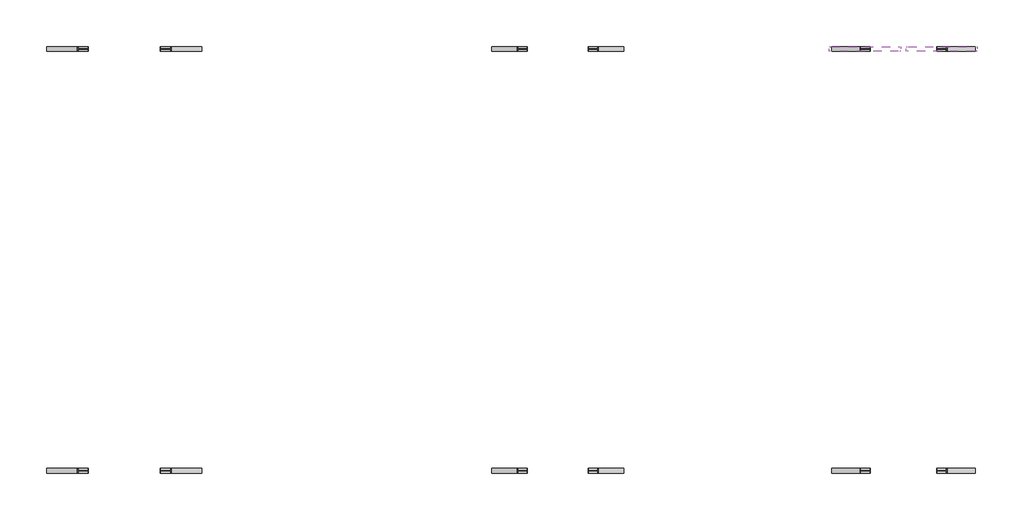
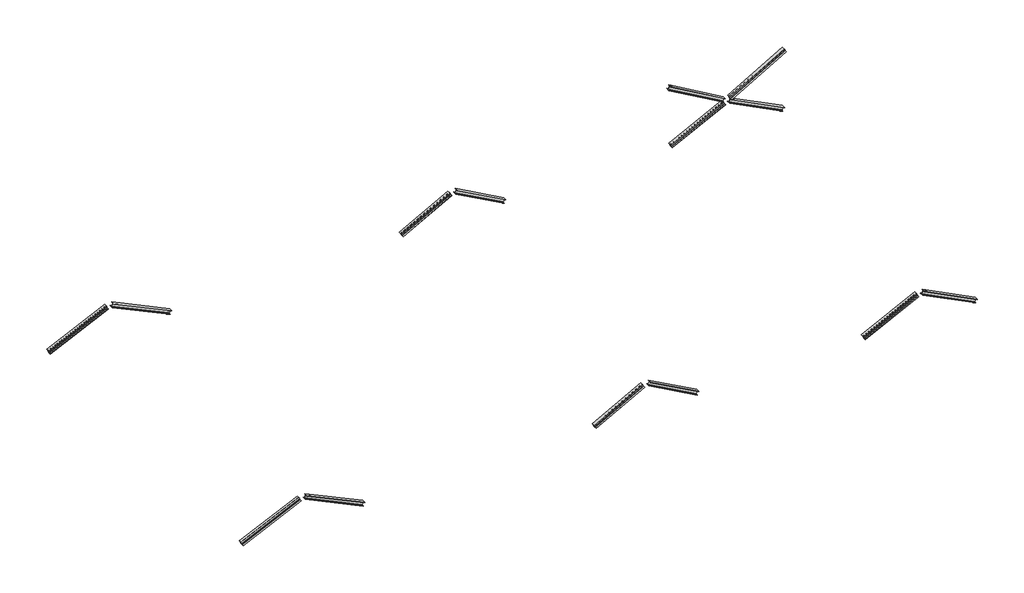
# One storey: 14 beams.
"""IFC4 building model written with IfcOpenShell, lengths in millimetres."""

import ifcopenshell
import ifcopenshell.guid

model = None  # the IFC model being written
_history = None  # IfcOwnerHistory: only IFC2X3 demands one
_inside = {}  # id of a spatial element -> (the spatial element, [elements in it])
_under = {}  # id of a project, library or spatial element -> (it, [spatial elements below it])
_declared = {}  # id of a project -> (the project, [libraries it declares])
_typed = {}  # id of a type object -> (the type object, [elements of that type])
_made_of = {}  # id of a material, layer set ... -> (it, [elements and type objects made of it])


def new_model(schema):
    """Start an empty IFC model of exactly this schema.

    Asked for "IFC4X3", IfcOpenShell would pick the latest addendum, in which some entities
    have other attributes; the version numbers below select the first issue.
    IFC2X3 requires an IfcOwnerHistory on every rooted entity: one is made here for all.
    """
    global model, _history
    if schema == "IFC4X3":
        model = ifcopenshell.file(schema_version=(4, 3, 0, 0))
    else:
        model = ifcopenshell.file(schema=schema)
    _inside.clear()
    _under.clear()
    _declared.clear()
    _typed.clear()
    _made_of.clear()
    _history = None
    if model.schema == "IFC2X3":
        org = make("IfcOrganization", Name="unknown")
        user = make(
            "IfcPersonAndOrganization",
            ThePerson=make("IfcPerson", FamilyName="unknown"),
            TheOrganization=org,
        )
        app = make(
            "IfcApplication",
            ApplicationDeveloper=org,
            Version="unknown",
            ApplicationFullName="unknown",
            ApplicationIdentifier="unknown",
        )
        _history = make(
            "IfcOwnerHistory",
            OwningUser=user,
            OwningApplication=app,
            ChangeAction="ADDED",
            CreationDate=0,
        )
    return model


def make(cls, **values):
    """One entity of the class cls with the attributes given. An attribute that is None is left unset."""
    return model.create_entity(
        cls, **{name: value for name, value in values.items() if value is not None}
    )


def rooted(cls, **values):
    """An entity with a GlobalId (a new one), such as an element, a storey or a relation."""
    return make(cls, GlobalId=ifcopenshell.guid.new(), OwnerHistory=_history, **values)


def si_unit(unit_type, name, prefix=None):
    """IfcSIUnit, for example si_unit("LENGTHUNIT", "METRE", prefix="MILLI")."""
    return make("IfcSIUnit", UnitType=unit_type, Prefix=prefix, Name=name)


def assignment(units):
    """IfcUnitAssignment: the units of a project."""
    return None if units is None else make("IfcUnitAssignment", Units=units)


def point(xyz):
    """IfcCartesianPoint."""
    return None if xyz is None else make("IfcCartesianPoint", Coordinates=xyz)


def direction(xyz):
    """IfcDirection."""
    return None if xyz is None else make("IfcDirection", DirectionRatios=xyz)


def frame(location, z_axis=None, x_axis=None):
    """IfcAxis2Placement3D, a coordinate frame: its origin and axes. An axis left out is left unset."""
    return make(
        "IfcAxis2Placement3D",
        Location=point(location),
        Axis=direction(z_axis),
        RefDirection=direction(x_axis),
    )


def frame_2d(location, x_axis=None):
    """IfcAxis2Placement2D, a coordinate frame in the plane: its origin and x axis."""
    return make(
        "IfcAxis2Placement2D", Location=point(location), RefDirection=direction(x_axis)
    )


def origin():
    """The frame at (0, 0, 0) with its axes left unset."""
    return frame((0.0, 0.0, 0.0))


def place(relative_to, where):
    """IfcLocalPlacement: puts the frame where relative to a parent placement (None: the world)."""
    return make(
        "IfcLocalPlacement", PlacementRelTo=relative_to, RelativePlacement=where
    )


def context(
    kind, dimensions, precision=None, world=None, true_north=None, identifier=None
):
    """IfcGeometricRepresentationContext, for example the 3D "Model" context."""
    return make(
        "IfcGeometricRepresentationContext",
        ContextIdentifier=identifier,
        ContextType=kind,
        CoordinateSpaceDimension=dimensions,
        Precision=precision,
        WorldCoordinateSystem=world,
        TrueNorth=true_north,
    )


def project(units=None, contexts=None):
    """IfcProject with its units and contexts."""
    return rooted(
        "IfcProject",
        Name="project",
        RepresentationContexts=contexts,
        UnitsInContext=assignment(units),
    )


def spatial(cls, under=None, at=None, **own):
    """A site, building, storey or space (cls), placed at a placement, below another one or the project."""
    s = rooted(cls, ObjectPlacement=at, **own)
    if under is not None:
        _under.setdefault(under.id(), (under, []))[1].append(s)
    return s


def polyline(points):
    """IfcPolyline through the points."""
    return make("IfcPolyline", Points=[point(p) for p in points])


def circle_curve(where, radius):
    """IfcCircle in the frame where."""
    return make("IfcCircle", Position=where, Radius=radius)


def trimmed(basis, trim1, trim2, sense, master):
    """IfcTrimmedCurve: the piece of a basis curve between two trims."""
    return make(
        "IfcTrimmedCurve",
        BasisCurve=basis,
        Trim1=trim1,
        Trim2=trim2,
        SenseAgreement=sense,
        MasterRepresentation=master,
    )


def segment(curve, same_sense, transition):
    """IfcCompositeCurveSegment."""
    return make(
        "IfcCompositeCurveSegment",
        Transition=transition,
        SameSense=same_sense,
        ParentCurve=curve,
    )


def composite_curve(segments, self_intersect=None):
    """IfcCompositeCurve: segments joined end to end."""
    return make("IfcCompositeCurve", Segments=segments, SelfIntersect=self_intersect)


def outline(outer, holes=None, kind="AREA"):
    """IfcArbitraryClosedProfileDef: a profile drawn as a closed curve; with holes, ...WithVoids."""
    if holes is None:
        return make("IfcArbitraryClosedProfileDef", ProfileType=kind, OuterCurve=outer)
    return make(
        "IfcArbitraryProfileDefWithVoids",
        ProfileType=kind,
        OuterCurve=outer,
        InnerCurves=holes,
    )


def extrude(swept, where, along, depth):
    """IfcExtrudedAreaSolid: the profile swept, set in the frame where, extruded along a direction by depth."""
    return make(
        "IfcExtrudedAreaSolid",
        SweptArea=swept,
        Position=where,
        ExtrudedDirection=direction(along),
        Depth=depth,
    )


def shape(context_of_items, identifier, shape_type, items):
    """IfcShapeRepresentation: the items that make up one representation, for example the "Body"."""
    return make(
        "IfcShapeRepresentation",
        ContextOfItems=context_of_items,
        RepresentationIdentifier=identifier,
        RepresentationType=shape_type,
        Items=items,
    )


def source(mapping_origin, context_of_items, identifier, shape_type, items):
    """IfcRepresentationMap: a shape defined once, which mapped items show again and again."""
    return make(
        "IfcRepresentationMap",
        MappingOrigin=mapping_origin,
        MappedRepresentation=shape(context_of_items, identifier, shape_type, items),
    )


def transform(
    local_origin,
    x_axis=None,
    y_axis=None,
    z_axis=None,
    scale=None,
    scale2=None,
    scale3=None,
    uniform=True,
):
    """IfcCartesianTransformationOperator3D, or its non-uniform kind. x_axis, y_axis, z_axis: its Axis1, 2, 3."""
    if uniform:
        return make(
            "IfcCartesianTransformationOperator3D",
            Axis1=direction(x_axis),
            Axis2=direction(y_axis),
            LocalOrigin=point(local_origin),
            Scale=scale,
            Axis3=direction(z_axis),
        )
    return make(
        "IfcCartesianTransformationOperator3DnonUniform",
        Axis1=direction(x_axis),
        Axis2=direction(y_axis),
        LocalOrigin=point(local_origin),
        Scale=scale,
        Axis3=direction(z_axis),
        Scale2=scale2,
        Scale3=scale3,
    )


def mapped(mapping_source, mapping_target):
    """IfcMappedItem: shows the shape of a source again, moved by a transform."""
    return make(
        "IfcMappedItem", MappingSource=mapping_source, MappingTarget=mapping_target
    )


def made_of(thing, what):
    """Note that an element or type object is made of a material, layer set ...; save() writes the relation."""
    if what is not None:
        _made_of.setdefault(what.id(), (what, []))[1].append(thing)
    return thing


def element(
    cls,
    number,
    at=None,
    inside=None,
    cuts=None,
    type_object=None,
    material=None,
    context=None,
    identifier="Body",
    shape_type=None,
    held_by="IfcProductDefinitionShape",
    body=None,
    shapes=None,
    **own,
):
    """One element of the class cls, such as IfcWall. Its Tag is "e" and its number.

    at: its placement. inside: the storey or other place that contains it. cuts: it is an
    opening in that element (IfcRelVoidsElement). A single representation is given by context,
    identifier, shape_type and body (its items); several are given by shapes. held_by: the class
    of the entity that holds the representations. save() writes the other relations.
    """
    e = rooted(cls, Tag="e%d" % number, ObjectPlacement=at, **own)
    if body is not None:
        shapes = [shape(context, identifier, shape_type, body)]
    if shapes is not None:
        e.Representation = make(held_by, Representations=shapes)
    if inside is not None:
        _inside.setdefault(inside.id(), (inside, []))[1].append(e)
    if cuts is not None:
        rooted(
            "IfcRelVoidsElement", RelatingBuildingElement=cuts, RelatedOpeningElement=e
        )
    if type_object is not None:
        _typed.setdefault(type_object.id(), (type_object, []))[1].append(e)
    return made_of(e, material)


def aggregate(whole, parts):
    """IfcRelAggregates: a whole, such as a stair, and the parts it consists of."""
    return rooted("IfcRelAggregates", RelatingObject=whole, RelatedObjects=parts)


def save(model, path):
    """Write the relations noted so far, then the file.

    IfcRelAggregates (storeys below a building ...), IfcRelContainedInSpatialStructure (elements
    in a storey), IfcRelDefinesByType, IfcRelAssociatesMaterial and IfcRelDeclares: one each for
    every whole, place, type object, material and project.
    """
    for whole, parts in _under.values():
        aggregate(whole, parts)
    for where, things in _inside.values():
        rooted(
            "IfcRelContainedInSpatialStructure",
            RelatedElements=things,
            RelatingStructure=where,
        )
    for kind, things in _typed.values():
        rooted("IfcRelDefinesByType", RelatedObjects=things, RelatingType=kind)
    for what, things in _made_of.values():
        rooted("IfcRelAssociatesMaterial", RelatedObjects=things, RelatingMaterial=what)
    for by, libraries in _declared.values():
        rooted("IfcRelDeclares", RelatingContext=by, RelatedDefinitions=libraries)
    model.write(path)


def beam_0eb71ca4(model_context):
    return source(origin(), model_context, "Body", "SweptSolid", [
        extrude(outline(composite_curve([segment(polyline([(100.0, -88.0), (100.0, -100.0), (-100.0, -100.0), (-100.0, -88.0), (-17.0, -88.0)]), True, "CONTINUOUS"), segment(trimmed(circle_curve(frame_2d((-17.0, -75.0)), 13.0), [point((-17.0, -88.0))], [point((-4.0, -75.0))], True, "CARTESIAN"), True, "CONTINUOUS"), segment(polyline([(-4.0, -75.0), (-4.0, 75.0)]), True, "CONTINUOUS"), segment(trimmed(circle_curve(frame_2d((-17.0, 75.0)), 13.0), [point((-4.0, 75.0))], [point((-17.0, 88.0))], True, "CARTESIAN"), True, "CONTINUOUS"), segment(polyline([(-17.0, 88.0), (-100.0, 88.0), (-100.0, 100.0), (100.0, 100.0), (100.0, 88.0), (17.0, 88.0)]), True, "CONTINUOUS"), segment(trimmed(circle_curve(frame_2d((17.0, 75.0)), 13.0), [point((17.0, 88.0))], [point((4.0, 75.0))], True, "CARTESIAN"), True, "CONTINUOUS"), segment(polyline([(4.0, 75.0), (4.0, -75.0)]), True, "CONTINUOUS"), segment(trimmed(circle_curve(frame_2d((17.0, -75.0)), 13.0), [point((4.0, -75.0))], [point((17.0, -88.0))], True, "CARTESIAN"), True, "CONTINUOUS"), segment(polyline([(17.0, -88.0), (100.0, -88.0)]), True, "CONTINUOUS")], self_intersect=False)), frame((-1683.7594404, 0.0, 0.0), z_axis=(1.0, 0.0, 0.0), x_axis=(0.0, 1.0, 0.0)), (0.0, 0.0, 1.0), 3450.380526),
    ])


def beam_a5566726(model_context):
    return source(origin(), model_context, "Body", "SweptSolid", [
        extrude(outline(composite_curve([segment(polyline([(100.0, -88.0), (100.0, -100.0), (-100.0, -100.0), (-100.0, -88.0), (-17.0, -88.0)]), True, "CONTINUOUS"), segment(trimmed(circle_curve(frame_2d((-17.0, -75.0)), 13.0), [point((-17.0, -88.0))], [point((-4.0, -75.0))], True, "CARTESIAN"), True, "CONTINUOUS"), segment(polyline([(-4.0, -75.0), (-4.0, 75.0)]), True, "CONTINUOUS"), segment(trimmed(circle_curve(frame_2d((-17.0, 75.0)), 13.0), [point((-4.0, 75.0))], [point((-17.0, 88.0))], True, "CARTESIAN"), True, "CONTINUOUS"), segment(polyline([(-17.0, 88.0), (-100.0, 88.0), (-100.0, 100.0), (100.0, 100.0), (100.0, 88.0), (17.0, 88.0)]), True, "CONTINUOUS"), segment(trimmed(circle_curve(frame_2d((17.0, 75.0)), 13.0), [point((17.0, 88.0))], [point((4.0, 75.0))], True, "CARTESIAN"), True, "CONTINUOUS"), segment(polyline([(4.0, 75.0), (4.0, -75.0)]), True, "CONTINUOUS"), segment(trimmed(circle_curve(frame_2d((17.0, -75.0)), 13.0), [point((4.0, -75.0))], [point((17.0, -88.0))], True, "CARTESIAN"), True, "CONTINUOUS"), segment(polyline([(17.0, -88.0), (100.0, -88.0)]), True, "CONTINUOUS")], self_intersect=False)), frame((-1443.5851857, 0.0, 0.0), z_axis=(1.0, 0.0, 0.0), x_axis=(0.0, 1.0, 0.0)), (0.0, 0.0, 1.0), 2972.6935261),
    ])


def beam_881e6142(model_context):
    return source(origin(), model_context, "Body", "SweptSolid", [
        extrude(outline(composite_curve([segment(polyline([(100.0, -88.0), (100.0, -100.0), (-100.0, -100.0), (-100.0, -88.0), (-17.0, -88.0)]), True, "CONTINUOUS"), segment(trimmed(circle_curve(frame_2d((-17.0, -75.0)), 13.0), [point((-17.0, -88.0))], [point((-4.0, -75.0))], True, "CARTESIAN"), True, "CONTINUOUS"), segment(polyline([(-4.0, -75.0), (-4.0, 75.0)]), True, "CONTINUOUS"), segment(trimmed(circle_curve(frame_2d((-17.0, 75.0)), 13.0), [point((-4.0, 75.0))], [point((-17.0, 88.0))], True, "CARTESIAN"), True, "CONTINUOUS"), segment(polyline([(-17.0, 88.0), (-100.0, 88.0), (-100.0, 100.0), (100.0, 100.0), (100.0, 88.0), (17.0, 88.0)]), True, "CONTINUOUS"), segment(trimmed(circle_curve(frame_2d((17.0, 75.0)), 13.0), [point((17.0, 88.0))], [point((4.0, 75.0))], True, "CARTESIAN"), True, "CONTINUOUS"), segment(polyline([(4.0, 75.0), (4.0, -75.0)]), True, "CONTINUOUS"), segment(trimmed(circle_curve(frame_2d((17.0, -75.0)), 13.0), [point((4.0, -75.0))], [point((17.0, -88.0))], True, "CARTESIAN"), True, "CONTINUOUS"), segment(polyline([(17.0, -88.0), (100.0, -88.0)]), True, "CONTINUOUS")], self_intersect=False)), frame((-1563.5376228, 0.0, 0.0), z_axis=(1.0, 0.0, 0.0), x_axis=(0.0, 1.0, 0.0)), (0.0, 0.0, 1.0), 3211.1247957),
    ])


def beam_623e387b(model_context):
    return source(origin(), model_context, "Body", "SweptSolid", [
        extrude(outline(composite_curve([segment(polyline([(-100.0, -88.0), (-17.0, -88.0)]), True, "CONTINUOUS"), segment(trimmed(circle_curve(frame_2d((-17.0, -75.0)), 13.0), [point((-17.0, -88.0))], [point((-4.0, -75.0))], True, "CARTESIAN"), True, "CONTINUOUS"), segment(polyline([(-4.0, -75.0), (-4.0, 75.0)]), True, "CONTINUOUS"), segment(trimmed(circle_curve(frame_2d((-17.0, 75.0)), 13.0), [point((-4.0, 75.0))], [point((-17.0, 88.0))], True, "CARTESIAN"), True, "CONTINUOUS"), segment(polyline([(-17.0, 88.0), (-100.0, 88.0), (-100.0, 100.0), (100.0, 100.0), (100.0, 88.0), (17.0, 88.0)]), True, "CONTINUOUS"), segment(trimmed(circle_curve(frame_2d((17.0, 75.0)), 13.0), [point((17.0, 88.0))], [point((4.0, 75.0))], True, "CARTESIAN"), True, "CONTINUOUS"), segment(polyline([(4.0, 75.0), (4.0, -75.0)]), True, "CONTINUOUS"), segment(trimmed(circle_curve(frame_2d((17.0, -75.0)), 13.0), [point((4.0, -75.0))], [point((17.0, -88.0))], True, "CARTESIAN"), True, "CONTINUOUS"), segment(polyline([(17.0, -88.0), (100.0, -88.0), (100.0, -100.0), (-100.0, -100.0), (-100.0, -88.0)]), True, "CONTINUOUS")], self_intersect=False)), frame((-1715.1887846, 0.0, 0.0), z_axis=(1.0, 0.0, 0.0), x_axis=(0.0, 1.0, 0.0)), (0.0, 0.0, 1.0), 3399.973917),
    ])


model = new_model("IFC4")

# Units and contexts
model_context = context("Model", 3, world=origin())
ifc_project = project(units=[si_unit("LENGTHUNIT", "METRE", prefix="MILLI")], contexts=[model_context])

# Site, building, storey
site = spatial("IfcSite", under=ifc_project)
building = spatial("IfcBuilding", under=site)
storey = spatial("IfcBuildingStorey", under=building, Name="G.L", Elevation=299.9720055)

# Beams
placement = place(None, origin())
beam_shape = beam_0eb71ca4(model_context)
element("IfcBeam", 1, ObjectType="0912_Steel Framing_H-KSD3502 : H_SB_ASB_H-200x200x8x12", at=placement, inside=storey, context=model_context, shape_type="MappedRepresentation", body=[
    mapped(beam_shape, transform((1750.0, 20999.5208589, 1507.9720055), x_axis=(0.9051232306684414, 0.0, 0.4251493117768432), y_axis=(0.0, 1.0, 0.0), z_axis=(-0.4251493117768432, 0.0, 0.9051232306684414))),
])
element("IfcBeam", 2, ObjectType="0912_Steel Framing_H-KSD3502 : H_SB_ASB_H-200x200x8x12", at=placement, inside=storey, context=model_context, shape_type="MappedRepresentation", body=[
    mapped(beam_shape, transform((5250.0, 20999.5208589, 1507.9720055), x_axis=(-0.9051232306684284, 0.0, 0.4251493117768708), y_axis=(0.0, -1.0, 0.0), z_axis=(0.4251493117768708, 0.0, 0.9051232306684284))),
])
element("IfcBeam", 3, ObjectType="0912_Steel Framing_H-KSD3502 : H_SB_ASB_H-200x200x8x12", at=placement, inside=storey, context=model_context, shape_type="MappedRepresentation", body=[
    mapped(beam_shape, transform((1750.0, 38999.5208589, 1507.9720055), x_axis=(0.9051232306684415, 0.0, 0.4251493117768429), y_axis=(0.0, 1.0, 0.0), z_axis=(-0.4251493117768429, 0.0, 0.9051232306684415))),
])
element("IfcBeam", 4, ObjectType="0912_Steel Framing_H-KSD3502 : H_SB_ASB_H-200x200x8x12", at=placement, inside=storey, context=model_context, shape_type="MappedRepresentation", body=[
    mapped(beam_shape, transform((5250.0, 38999.5208589, 1507.9720055), x_axis=(-0.9051232306684285, 0.0, 0.4251493117768706), y_axis=(0.0, -1.0, 0.0), z_axis=(0.4251493117768706, 0.0, 0.9051232306684285))),
])
beam_2_shape = beam_a5566726(model_context)
element("IfcBeam", 5, ObjectType="0912_Steel Framing_H-KSD3502 : H_SB_ASB_H-200x200x8x12", at=placement, inside=storey, context=model_context, shape_type="MappedRepresentation", body=[
    mapped(beam_2_shape, transform((20500.0, 20999.5208589, 1507.9720055), x_axis=(0.8769554889666458, 0.0, 0.4805716079537693), y_axis=(0.0, 1.0, 0.0), z_axis=(-0.4805716079537693, 0.0, 0.8769554889666458))),
])
element("IfcBeam", 6, ObjectType="0912_Steel Framing_H-KSD3502 : H_SB_ASB_H-200x200x8x12", at=placement, inside=storey, context=model_context, shape_type="MappedRepresentation", body=[
    mapped(beam_2_shape, transform((23500.0, 20999.5208589, 1507.9720055), x_axis=(-0.8769554889666746, 0.0, 0.4805716079537164), y_axis=(0.0, -1.0, 0.0), z_axis=(0.4805716079537164, 0.0, 0.8769554889666746))),
])
element("IfcBeam", 7, ObjectType="0912_Steel Framing_H-KSD3502 : H_SB_ASB_H-200x200x8x12", at=placement, inside=storey, context=model_context, shape_type="MappedRepresentation", body=[
    mapped(beam_2_shape, transform((20500.0, 38999.5208589, 1507.9720055), x_axis=(0.8769554889666475, 0.0, 0.4805716079537661), y_axis=(0.0, 1.0, 0.0), z_axis=(-0.4805716079537661, 0.0, 0.8769554889666475))),
])
element("IfcBeam", 8, ObjectType="0912_Steel Framing_H-KSD3502 : H_SB_ASB_H-200x200x8x12", at=placement, inside=storey, context=model_context, shape_type="MappedRepresentation", body=[
    mapped(beam_2_shape, transform((23500.0, 38999.5208589, 1507.9720055), x_axis=(-0.8769554889666732, 0.0, 0.4805716079537191), y_axis=(0.0, -1.0, 0.0), z_axis=(0.4805716079537191, 0.0, 0.8769554889666732))),
])
beam_3_shape = beam_881e6142(model_context)
element("IfcBeam", 9, ObjectType="0912_Steel Framing_H-KSD3502 : H_SB_ASB_H-200x200x8x12", at=placement, inside=storey, context=model_context, shape_type="MappedRepresentation", body=[
    mapped(beam_3_shape, transform((38375.0, 20999.5208589, 1507.9720055), x_axis=(-0.8923307733807315, 0.0, 0.4513820896732006), y_axis=(0.0, -1.0, 0.0), z_axis=(0.4513820896732006, 0.0, 0.8923307733807315))),
])
element("IfcBeam", 10, ObjectType="0912_Steel Framing_H-KSD3502 : H_SB_ASB_H-200x200x8x12", at=placement, inside=storey, context=model_context, shape_type="MappedRepresentation", body=[
    mapped(beam_3_shape, transform((35125.0, 20999.5208589, 1507.9720055), x_axis=(0.8923307733807281, 0.0, 0.45138208967320764), y_axis=(0.0, 1.0, 0.0), z_axis=(-0.45138208967320764, 0.0, 0.8923307733807281))),
])
element("IfcBeam", 11, ObjectType="0912_Steel Framing_H-KSD3502 : H_SB_ASB_H-200x200x8x12", at=placement, inside=storey, context=model_context, shape_type="MappedRepresentation", body=[
    mapped(beam_3_shape, transform((38375.0, 38999.5208589, 1507.9720055), x_axis=(-0.8923307733807311, 0.0, 0.45138208967320154), y_axis=(0.0, -1.0, 0.0), z_axis=(0.45138208967320154, 0.0, 0.8923307733807311))),
])
element("IfcBeam", 12, ObjectType="0912_Steel Framing_H-KSD3502 : H_SB_ASB_H-200x200x8x12", at=placement, inside=storey, context=model_context, shape_type="MappedRepresentation", body=[
    mapped(beam_3_shape, transform((35125.0, 38999.5208589, 1507.9720055), x_axis=(0.8923307733807282, 0.0, 0.4513820896732074), y_axis=(0.0, 1.0, 0.0), z_axis=(-0.4513820896732074, 0.0, 0.8923307733807282))),
])
beam_4_shape = beam_623e387b(model_context)
element("IfcBeam", 13, ObjectType="0912_Steel Framing_H-KSD3502 : H_SB_ASB_H-200x200x8x12", at=placement, inside=storey, context=model_context, shape_type="MappedRepresentation", body=[
    mapped(beam_4_shape, transform((38375.0, 38999.5208589, 3269.4720055), x_axis=(-0.8657240101232682, 0.0, -0.5005216661605044), y_axis=(0.0, -1.0, 0.0), z_axis=(-0.5005216661605044, 0.0, 0.8657240101232682))),
])
element("IfcBeam", 14, ObjectType="0912_Steel Framing_H-KSD3502 : H_SB_ASB_H-200x200x8x12", at=placement, inside=storey, context=model_context, shape_type="MappedRepresentation", body=[
    mapped(beam_4_shape, transform((35125.0, 38999.5208589, 3269.4720055), x_axis=(0.8657240101232683, 0.0, -0.5005216661605043), y_axis=(0.0, 1.0, 0.0), z_axis=(0.5005216661605043, 0.0, 0.8657240101232683))),
])

save(model, "model.ifc")

# Revit data of these elements
# Type "0912_Steel Framing_H-KSD3502 : H_SB_ASB_H-200x200x8x12"
#   H_WM Code_1 = "S01AA002-00001 | Main Steel Structure Fabrication Work | Shelter/Building | Medium Steel - Standard (90KG/M>Weight≥30KG/M) | Material: (   )"
#   H_WM Code_2 = "S03AA028-00001 | Main Steel Structure Erection Work | Shelter/Building | Medium Steel (90KG/M>Weight≥30KG/M) | Material: (   )"
#   H_WM Code_3 = "S01AA010-00001 | Main Steel Structure Fabrication Work | Shelter/Building | Steel Painting/Coating | for Non-Fireproofed Steel Surface, Surface Preparation, Primer, Second & Final Coat | Material: (   )"
#   H_Q'ty Cal Type Tag = "SB-Q2"
#   Width = 20.0 cm
#   Web Thickness = 0.8 cm
#   Web Fillet = 1.3 cm
#   Warping Constant = 141000.0 cm⁶
#   W = 0
#   Torsional Moment of Inertia = 26.2485 cm⁴
#   Section Area = 63.53 cm²
#   Plastic Modulus weak axis = 244.0 cm³
#   Plastic Modulus strong axis = 525.0 cm³
#   Perimeter = 1.16 m²/m
#   Nominal Weight = 49.90 kgf/m
#   Moment of Inertia weak axis = 1600.00 cm⁴
#   Moment of Inertia strong axis = 4720.00 cm⁴
#   Height = 20.0 cm
#   Flange Thickness = 1.2 cm
#   Elastic Modulus weak axis = 160.0 cm³
#   Elastic Modulus strong axis = 472.0 cm³
#   Centroid Vertical = 10.0 cm
#   Centroid Horizontal = 10.0 cm
#   Ix = 47200000
#   Length [instance default] = 1.5240 m
#   Zx = 525000
#   b = 0.2000 m
#   h = 0.2000 m
#   r = 0.0130 m
#   s = 0.0080 m
#   t = 0.0120 m
#   A = 0.006353 m²
#   Structural Material [instance default] = Steel, 45-345
#   Assembly Code = ""
# Elements 1, 2, 5, 6, 9, 10 (IfcBeam, "0912_Steel Framing_H-KSD3502 : H_SB_ASB_H-200x200x8x12")
#   Mark = "VB1"
#   LINE SCHEDULE = "A"
#   Structural Material = none
#   Phase Created = New Construction
# Elements 3, 4, 7, 8, 11, 12, 13, 14 (IfcBeam, "0912_Steel Framing_H-KSD3502 : H_SB_ASB_H-200x200x8x12")
#   Mark = "VB1"
#   Structural Material = none
#   Phase Created = New Construction
# Materials
#   "Steel, 45-345": class "Metal", colour RGB 189 187 185, transparency 0, Description = "Steel 345 MPa", Cost = 0
